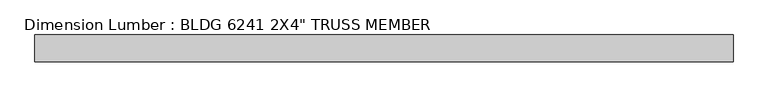
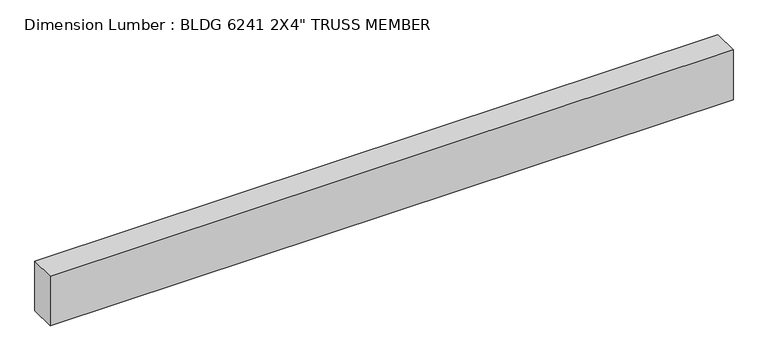
"""IFC4 building model written with IfcOpenShell, lengths in millimetres: beam geometry."""

import ifcopenshell
import ifcopenshell.guid

model = None  # the IFC model being written
_history = None  # IfcOwnerHistory: only IFC2X3 demands one
_inside = {}  # id of a spatial element -> (the spatial element, [elements in it])
_under = {}  # id of a project, library or spatial element -> (it, [spatial elements below it])
_declared = {}  # id of a project -> (the project, [libraries it declares])
_typed = {}  # id of a type object -> (the type object, [elements of that type])
_made_of = {}  # id of a material, layer set ... -> (it, [elements and type objects made of it])


def new_model(schema):
    """Start an empty IFC model of exactly this schema.

    Asked for "IFC4X3", IfcOpenShell would pick the latest addendum, in which some entities
    have other attributes; the version numbers below select the first issue.
    IFC2X3 requires an IfcOwnerHistory on every rooted entity: one is made here for all.
    """
    global model, _history
    if schema == "IFC4X3":
        model = ifcopenshell.file(schema_version=(4, 3, 0, 0))
    else:
        model = ifcopenshell.file(schema=schema)
    _inside.clear()
    _under.clear()
    _declared.clear()
    _typed.clear()
    _made_of.clear()
    _history = None
    if model.schema == "IFC2X3":
        org = make("IfcOrganization", Name="unknown")
        user = make(
            "IfcPersonAndOrganization",
            ThePerson=make("IfcPerson", FamilyName="unknown"),
            TheOrganization=org,
        )
        app = make(
            "IfcApplication",
            ApplicationDeveloper=org,
            Version="unknown",
            ApplicationFullName="unknown",
            ApplicationIdentifier="unknown",
        )
        _history = make(
            "IfcOwnerHistory",
            OwningUser=user,
            OwningApplication=app,
            ChangeAction="ADDED",
            CreationDate=0,
        )
    return model


def make(cls, **values):
    """One entity of the class cls with the attributes given. An attribute that is None is left unset."""
    return model.create_entity(
        cls, **{name: value for name, value in values.items() if value is not None}
    )


def rooted(cls, **values):
    """An entity with a GlobalId (a new one), such as an element, a storey or a relation."""
    return make(cls, GlobalId=ifcopenshell.guid.new(), OwnerHistory=_history, **values)


def si_unit(unit_type, name, prefix=None):
    """IfcSIUnit, for example si_unit("LENGTHUNIT", "METRE", prefix="MILLI")."""
    return make("IfcSIUnit", UnitType=unit_type, Prefix=prefix, Name=name)


def assignment(units):
    """IfcUnitAssignment: the units of a project."""
    return None if units is None else make("IfcUnitAssignment", Units=units)


def point(xyz):
    """IfcCartesianPoint."""
    return None if xyz is None else make("IfcCartesianPoint", Coordinates=xyz)


def direction(xyz):
    """IfcDirection."""
    return None if xyz is None else make("IfcDirection", DirectionRatios=xyz)


def frame(location, z_axis=None, x_axis=None):
    """IfcAxis2Placement3D, a coordinate frame: its origin and axes. An axis left out is left unset."""
    return make(
        "IfcAxis2Placement3D",
        Location=point(location),
        Axis=direction(z_axis),
        RefDirection=direction(x_axis),
    )


def origin():
    """The frame at (0, 0, 0) with its axes left unset."""
    return frame((0.0, 0.0, 0.0))


def place(relative_to, where):
    """IfcLocalPlacement: puts the frame where relative to a parent placement (None: the world)."""
    return make(
        "IfcLocalPlacement", PlacementRelTo=relative_to, RelativePlacement=where
    )


def context(
    kind, dimensions, precision=None, world=None, true_north=None, identifier=None
):
    """IfcGeometricRepresentationContext, for example the 3D "Model" context."""
    return make(
        "IfcGeometricRepresentationContext",
        ContextIdentifier=identifier,
        ContextType=kind,
        CoordinateSpaceDimension=dimensions,
        Precision=precision,
        WorldCoordinateSystem=world,
        TrueNorth=true_north,
    )


def project(units=None, contexts=None):
    """IfcProject with its units and contexts."""
    return rooted(
        "IfcProject",
        Name="project",
        RepresentationContexts=contexts,
        UnitsInContext=assignment(units),
    )


def spatial(cls, under=None, at=None, **own):
    """A site, building, storey or space (cls), placed at a placement, below another one or the project."""
    s = rooted(cls, ObjectPlacement=at, **own)
    if under is not None:
        _under.setdefault(under.id(), (under, []))[1].append(s)
    return s


def polyline(points):
    """IfcPolyline through the points."""
    return make("IfcPolyline", Points=[point(p) for p in points])


def outline(outer, holes=None, kind="AREA"):
    """IfcArbitraryClosedProfileDef: a profile drawn as a closed curve; with holes, ...WithVoids."""
    if holes is None:
        return make("IfcArbitraryClosedProfileDef", ProfileType=kind, OuterCurve=outer)
    return make(
        "IfcArbitraryProfileDefWithVoids",
        ProfileType=kind,
        OuterCurve=outer,
        InnerCurves=holes,
    )


def extrude(swept, where, along, depth):
    """IfcExtrudedAreaSolid: the profile swept, set in the frame where, extruded along a direction by depth."""
    return make(
        "IfcExtrudedAreaSolid",
        SweptArea=swept,
        Position=where,
        ExtrudedDirection=direction(along),
        Depth=depth,
    )


def shape(context_of_items, identifier, shape_type, items):
    """IfcShapeRepresentation: the items that make up one representation, for example the "Body"."""
    return make(
        "IfcShapeRepresentation",
        ContextOfItems=context_of_items,
        RepresentationIdentifier=identifier,
        RepresentationType=shape_type,
        Items=items,
    )


def source(mapping_origin, context_of_items, identifier, shape_type, items):
    """IfcRepresentationMap: a shape defined once, which mapped items show again and again."""
    return make(
        "IfcRepresentationMap",
        MappingOrigin=mapping_origin,
        MappedRepresentation=shape(context_of_items, identifier, shape_type, items),
    )


def transform(
    local_origin,
    x_axis=None,
    y_axis=None,
    z_axis=None,
    scale=None,
    scale2=None,
    scale3=None,
    uniform=True,
):
    """IfcCartesianTransformationOperator3D, or its non-uniform kind. x_axis, y_axis, z_axis: its Axis1, 2, 3."""
    if uniform:
        return make(
            "IfcCartesianTransformationOperator3D",
            Axis1=direction(x_axis),
            Axis2=direction(y_axis),
            LocalOrigin=point(local_origin),
            Scale=scale,
            Axis3=direction(z_axis),
        )
    return make(
        "IfcCartesianTransformationOperator3DnonUniform",
        Axis1=direction(x_axis),
        Axis2=direction(y_axis),
        LocalOrigin=point(local_origin),
        Scale=scale,
        Axis3=direction(z_axis),
        Scale2=scale2,
        Scale3=scale3,
    )


def mapped(mapping_source, mapping_target):
    """IfcMappedItem: shows the shape of a source again, moved by a transform."""
    return make(
        "IfcMappedItem", MappingSource=mapping_source, MappingTarget=mapping_target
    )


def made_of(thing, what):
    """Note that an element or type object is made of a material, layer set ...; save() writes the relation."""
    if what is not None:
        _made_of.setdefault(what.id(), (what, []))[1].append(thing)
    return thing


def element(
    cls,
    number,
    at=None,
    inside=None,
    cuts=None,
    type_object=None,
    material=None,
    context=None,
    identifier="Body",
    shape_type=None,
    held_by="IfcProductDefinitionShape",
    body=None,
    shapes=None,
    **own,
):
    """One element of the class cls, such as IfcWall. Its Tag is "e" and its number.

    at: its placement. inside: the storey or other place that contains it. cuts: it is an
    opening in that element (IfcRelVoidsElement). A single representation is given by context,
    identifier, shape_type and body (its items); several are given by shapes. held_by: the class
    of the entity that holds the representations. save() writes the other relations.
    """
    e = rooted(cls, Tag="e%d" % number, ObjectPlacement=at, **own)
    if body is not None:
        shapes = [shape(context, identifier, shape_type, body)]
    if shapes is not None:
        e.Representation = make(held_by, Representations=shapes)
    if inside is not None:
        _inside.setdefault(inside.id(), (inside, []))[1].append(e)
    if cuts is not None:
        rooted(
            "IfcRelVoidsElement", RelatingBuildingElement=cuts, RelatedOpeningElement=e
        )
    if type_object is not None:
        _typed.setdefault(type_object.id(), (type_object, []))[1].append(e)
    return made_of(e, material)


def aggregate(whole, parts):
    """IfcRelAggregates: a whole, such as a stair, and the parts it consists of."""
    return rooted("IfcRelAggregates", RelatingObject=whole, RelatedObjects=parts)


def save(model, path):
    """Write the relations noted so far, then the file.

    IfcRelAggregates (storeys below a building ...), IfcRelContainedInSpatialStructure (elements
    in a storey), IfcRelDefinesByType, IfcRelAssociatesMaterial and IfcRelDeclares: one each for
    every whole, place, type object, material and project.
    """
    for whole, parts in _under.values():
        aggregate(whole, parts)
    for where, things in _inside.values():
        rooted(
            "IfcRelContainedInSpatialStructure",
            RelatedElements=things,
            RelatingStructure=where,
        )
    for kind, things in _typed.values():
        rooted("IfcRelDefinesByType", RelatedObjects=things, RelatingType=kind)
    for what, things in _made_of.values():
        rooted("IfcRelAssociatesMaterial", RelatedObjects=things, RelatingMaterial=what)
    for by, libraries in _declared.values():
        rooted("IfcRelDeclares", RelatingContext=by, RelatedDefinitions=libraries)
    model.write(path)


def beam_ec20356b(model_context):
    return source(origin(), model_context, "Body", "SweptSolid", [
        extrude(outline(polyline([(660.3999994, 25.4), (660.3999994, -25.4), (-660.3999994, -25.4), (-660.3999994, 25.4), (660.3999994, 25.4)])), frame((0.0, 0.0, -50.8), z_axis=(0.0, 0.0, 1.0), x_axis=(1.0, 0.0, 0.0)), (0.0, 0.0, 1.0), 101.6),
    ])


if __name__ == "__main__":
    model = new_model("IFC4")
    model_context = context("Model", 3, world=origin())
    ifc_project = project(units=[si_unit("LENGTHUNIT", "METRE", prefix="MILLI")], contexts=[model_context])
    site = spatial("IfcSite", under=ifc_project)
    building = spatial("IfcBuilding", under=site)
    placement = place(None, origin())
    beam_shape = beam_ec20356b(model_context)
    element("IfcBeam", 1, ObjectType="Dimension Lumber : BLDG 6241 2X4\" TRUSS MEMBER", at=placement, inside=building, context=model_context, shape_type="MappedRepresentation", body=[
        mapped(beam_shape, transform((0.0, 0.0, 0.0), x_axis=(1.0, 0.0, 0.0), y_axis=(0.0, 1.0, 0.0), z_axis=(0.0, 0.0, 1.0))),
    ])
    save(model, "model.ifc")

# Revit data of these elements
# Type "Dimension Lumber : BLDG 6241 2X4\" TRUSS MEMBER"
#   Assembly Code = "B10"
#   A = 0.273472 SF
#   Length [instance default] = 5' - 0"
#   b = 0' - 2"
#   d = 0' - 4"
#   Structural Material [instance default] = Softwood, Lumber
# Element 1 (IfcBeam, "Dimension Lumber : BLDG 6241 2X4\" TRUSS MEMBER")
#   Materials on its faces: "Softwood, Lumber"
# Materials
#   "Softwood, Lumber": class "Wood", colour RGB 223 192 134, transparency 0, Description = "Pinus Echinata", Cost = 0
